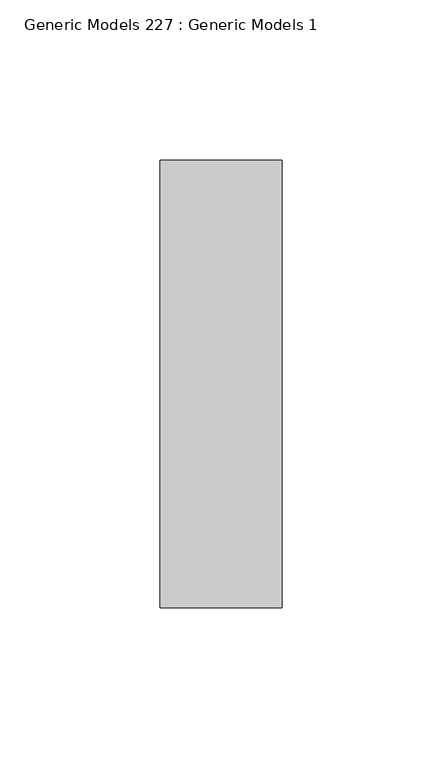
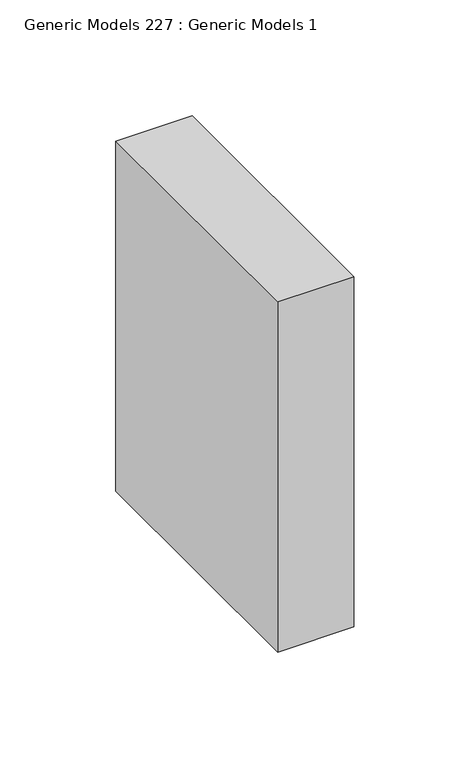
"""IFC4 building model written with IfcOpenShell, lengths in millimetres: proxy geometry, Generic Models 227 : Generic Models 1."""

from ifc_helpers import new_model, si_unit, frame, origin, place, context, project, spatial, polyline, outline, extrude, source, transform, mapped, element, save


def generic_models_227_generic_models_1_7f31316c(model_context):
    return source(origin(), model_context, "Body", "SweptSolid", [
        extrude(outline(polyline([(-13578.5613975, -29205.0985041), (-13578.5613975, -29344.7985041), (-13616.6613975, -29344.7985041), (-13616.6613975, -29205.0985041), (-13578.5613975, -29205.0985041)])), frame((0.0, 0.0, 126860.046), z_axis=(0.0, 0.0, 1.0), x_axis=(1.0, 0.0, 0.0)), (0.0, 0.0, 1.0), 184.6825599),
    ])


if __name__ == "__main__":
    model = new_model("IFC4")
    model_context = context("Model", 3, world=origin())
    ifc_project = project(units=[si_unit("LENGTHUNIT", "METRE", prefix="MILLI")], contexts=[model_context])
    site = spatial("IfcSite", under=ifc_project)
    building = spatial("IfcBuilding", under=site)
    placement = place(None, origin())
    generic_models_227_generic_models_1_shape = generic_models_227_generic_models_1_7f31316c(model_context)
    element("IfcBuildingElementProxy", 1, Name="Generic Models 227 : Generic Models 1", ObjectType="Generic Models 227 : Generic Models 1", at=placement, inside=building, context=model_context, shape_type="MappedRepresentation", body=[
        mapped(generic_models_227_generic_models_1_shape, transform((0.0, 0.0, 0.0), x_axis=(1.0, 0.0, 0.0), y_axis=(0.0, 1.0, 0.0), z_axis=(0.0, 0.0, 1.0))),
    ])
    save(model, "model.ifc")

# Revit data of these elements
# Element 1 (IfcBuildingElementProxy, "Generic Models 227 : Generic Models 1")
#   Materials on its faces: "_2X BLOCKING AS REQUIRED"
# Materials
#   "_2X BLOCKING AS REQUIRED": class "Generic", colour RGB 177 130 114, transparency 0, Cost = 0
